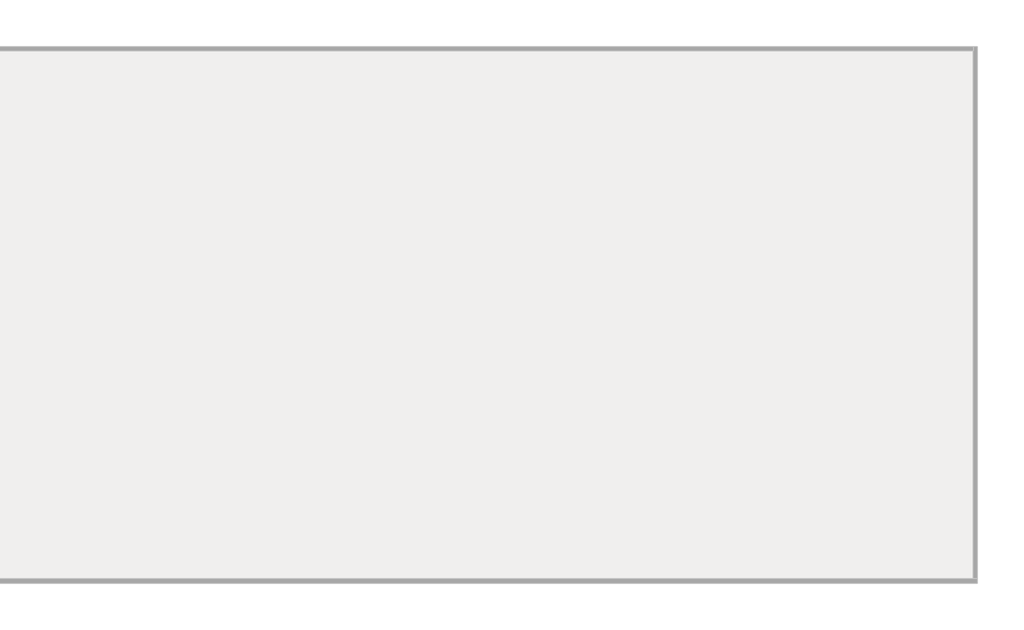
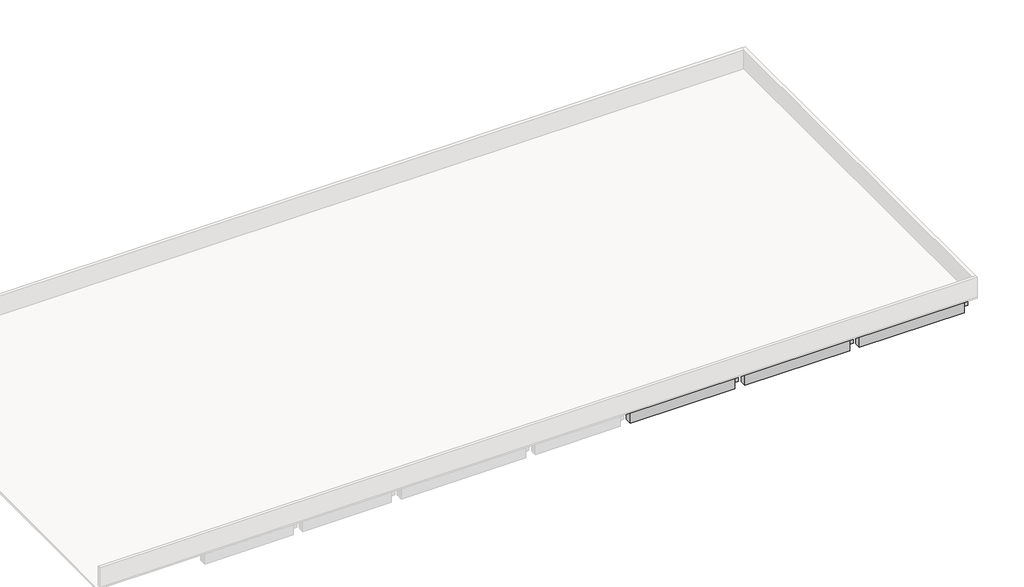
# One storey, part 2 of 2: 26 beams.
"""IFC4 building model written with IfcOpenShell, lengths in millimetres."""

from ifc_helpers import new_model, si_unit, origin, place, context, project, spatial, faceted_brep, element, save

model = new_model("IFC4")

# Units and contexts
model_context = context("Model", 3, world=origin())
ifc_project = project(units=[si_unit("LENGTHUNIT", "METRE", prefix="MILLI")], contexts=[model_context])

# Site, building, storey
site = spatial("IfcSite", under=ifc_project)
building = spatial("IfcBuilding", under=site)
storey = spatial("IfcBuildingStorey", under=building, Name="TOC", Elevation=7650.0)

# Beams
placement = place(None, origin())
element("IfcBeam", 1, ObjectType="RC Beam_Rectangular : H_SB_ACB_B400xH900", at=placement, inside=storey, context=model_context, shape_type="Brep", body=[
    faceted_brep([(39124.7, 12116.5208589, 6750.0), (39124.7, 12116.5208589, 7549.0), (38724.7, 12116.5208589, 7549.0), (33391.7, 12116.5208589, 7549.0), (33157.7, 12116.5208589, 7549.0), (32124.7, 12116.5208589, 7549.0), (32124.7, 12116.5208589, 6750.0), (33157.7, 12116.5208589, 6750.0), (33391.7, 12116.5208589, 6750.0), (38724.7, 12116.5208589, 6750.0), (39124.7, 12516.5208589, 6750.0), (32124.7, 12516.5208589, 6750.0), (33157.7, 12516.5208589, 6750.0), (33391.7, 12516.5208589, 6750.0), (38724.7, 12516.5208589, 6750.0), (39124.7, 12516.5208589, 7549.0), (32124.7, 12516.5208589, 7549.0), (33157.7, 12516.5208589, 7549.0), (33391.7, 12516.5208589, 7549.0), (38724.7, 12516.5208589, 7549.0)], [[[0, 1, 2, 3, 4, 5, 6, 7, 8, 9]], [[10, 0, 9, 8, 7, 6, 11, 12, 13, 14]], [[15, 10, 14, 13, 12, 11, 16, 17, 18, 19]], [[1, 15, 19, 18, 17, 16, 5, 4, 3, 2]], [[0, 10, 15, 1]], [[6, 5, 16, 11]]]),
])
element("IfcBeam", 2, ObjectType="RC Beam_Rectangular : H_SB_ACB_B400xH900", at=placement, inside=storey, context=model_context, shape_type="Brep", body=[
    faceted_brep([(46124.7, 12116.5208589, 6750.0), (46124.7, 12116.5208589, 7549.0), (45724.7, 12116.5208589, 7549.0), (43841.7, 12116.5208589, 7549.0), (43607.7, 12116.5208589, 7549.0), (39124.7, 12116.5208589, 7549.0), (39124.7, 12116.5208589, 6750.0), (43607.7, 12116.5208589, 6750.0), (43841.7, 12116.5208589, 6750.0), (45724.7, 12116.5208589, 6750.0), (46124.7, 12516.5208589, 6750.0), (39124.7, 12516.5208589, 6750.0), (43607.7, 12516.5208589, 6750.0), (43841.7, 12516.5208589, 6750.0), (45724.7, 12516.5208589, 6750.0), (46124.7, 12516.5208589, 7549.0), (39124.7, 12516.5208589, 7549.0), (43607.7, 12516.5208589, 7549.0), (43841.7, 12516.5208589, 7549.0), (45724.7, 12516.5208589, 7549.0)], [[[0, 1, 2, 3, 4, 5, 6, 7, 8, 9]], [[10, 0, 9, 8, 7, 6, 11, 12, 13, 14]], [[15, 10, 14, 13, 12, 11, 16, 17, 18, 19]], [[1, 15, 19, 18, 17, 16, 5, 4, 3, 2]], [[0, 10, 15, 1]], [[6, 5, 16, 11]]]),
])
element("IfcBeam", 3, ObjectType="RC Beam_Rectangular : H_SB_ACB_B400xH900", at=placement, inside=storey, context=model_context, shape_type="Brep", body=[
    faceted_brep([(53124.7, 12116.5208589, 6750.0), (53124.7, 12116.5208589, 7549.0), (52724.7, 12116.5208589, 7549.0), (46124.7, 12116.5208589, 7549.0), (46124.7, 12116.5208589, 6750.0), (52724.7, 12116.5208589, 6750.0), (53124.7, 12516.5208589, 6750.0), (46124.7, 12516.5208589, 6750.0), (52724.7, 12516.5208589, 6750.0), (53124.7, 12516.5208589, 7549.0), (46124.7, 12516.5208589, 7549.0), (52724.7, 12516.5208589, 7549.0)], [[[0, 1, 2, 3, 4, 5]], [[6, 0, 5, 4, 7, 8]], [[9, 6, 8, 7, 10, 11]], [[1, 9, 11, 10, 3, 2]], [[0, 6, 9, 1]], [[4, 3, 10, 7]]]),
])
element("IfcBeam", 4, ObjectType="RC Beam_Rectangular : H_SB_ACB_B400xH900", at=placement, inside=storey, context=model_context, shape_type="Brep", body=[
    faceted_brep([(18224.7, 23816.5208589, 7500.0), (18224.7, 23816.5208589, 6750.0), (25824.7, 23816.5208589, 6750.0), (25824.7, 23816.5208589, 7500.0), (25924.7, 23816.5208589, 7500.0), (25924.7, 23816.5208589, 7549.0), (18124.7, 23816.5208589, 7549.0), (18124.7, 23816.5208589, 7500.0), (18224.7, 23886.5208589, 6750.0), (18224.7, 24216.5208589, 6750.0), (25824.7, 24216.5208589, 6750.0), (25824.7, 23886.5208589, 6750.0), (18224.7, 24216.5208589, 7500.0), (18124.7, 24216.5208589, 7500.0), (18124.7, 24216.5208589, 7549.0), (25924.7, 24216.5208589, 7549.0), (25924.7, 24216.5208589, 7500.0), (25824.7, 24216.5208589, 7500.0)], [[[0, 1, 2, 3, 4, 5, 6, 7]], [[1, 8, 9, 10, 11, 2]], [[9, 12, 13, 14, 15, 16, 17, 10]], [[1, 0, 12, 9, 8]], [[0, 7, 13, 12]], [[3, 2, 11, 10, 17]], [[3, 17, 16, 4]], [[14, 6, 5, 15]], [[6, 14, 13, 7]], [[5, 4, 16, 15]]]),
])
element("IfcBeam", 5, ObjectType="RC Beam_Rectangular : H_SB_ACB_B400xH900", at=placement, inside=storey, context=model_context, shape_type="Brep", body=[
    faceted_brep([(26424.7, 23816.5208589, 7500.0), (26424.7, 23816.5208589, 6750.0), (31624.7, 23816.5208589, 6750.0), (31624.7, 23816.5208589, 7500.0), (31724.7, 23816.5208589, 7500.0), (31724.7, 23816.5208589, 7549.0), (26324.7, 23816.5208589, 7549.0), (26324.7, 23816.5208589, 7500.0), (26424.7, 23886.5208589, 6750.0), (26424.7, 24216.5208589, 6750.0), (31624.7, 24216.5208589, 6750.0), (31624.7, 23886.5208589, 6750.0), (26424.7, 24216.5208589, 7500.0), (26324.7, 24216.5208589, 7500.0), (26324.7, 24216.5208589, 7549.0), (31724.7, 24216.5208589, 7549.0), (31724.7, 24216.5208589, 7500.0), (31624.7, 24216.5208589, 7500.0)], [[[0, 1, 2, 3, 4, 5, 6, 7]], [[1, 8, 9, 10, 11, 2]], [[9, 12, 13, 14, 15, 16, 17, 10]], [[1, 0, 12, 9, 8]], [[0, 7, 13, 12]], [[3, 2, 11, 10, 17]], [[3, 17, 16, 4]], [[14, 6, 5, 15]], [[6, 14, 13, 7]], [[5, 4, 16, 15]]]),
])
element("IfcBeam", 6, ObjectType="RC Beam_Rectangular : H_SB_ACB_B400xH900", at=placement, inside=storey, context=model_context, shape_type="Brep", body=[
    faceted_brep([(32224.7, 23816.5208589, 7500.0), (32224.7, 23816.5208589, 6750.0), (33157.7, 23816.5208589, 6750.0), (33391.7, 23816.5208589, 6750.0), (38624.7, 23816.5208589, 6750.0), (38624.7, 23816.5208589, 7500.0), (38724.7, 23816.5208589, 7500.0), (38724.7, 23816.5208589, 7549.0), (33391.7, 23816.5208589, 7549.0), (33157.7, 23816.5208589, 7549.0), (32124.7, 23816.5208589, 7549.0), (32124.7, 23816.5208589, 7500.0), (32224.7, 23886.5208589, 6750.0), (32224.7, 24216.5208589, 6750.0), (38624.7, 24216.5208589, 6750.0), (38624.7, 23886.5208589, 6750.0), (32224.7, 24216.5208589, 7500.0), (32124.7, 24216.5208589, 7500.0), (32124.7, 24216.5208589, 7549.0), (38724.7, 24216.5208589, 7549.0), (38724.7, 24216.5208589, 7500.0), (38624.7, 24216.5208589, 7500.0)], [[[0, 1, 2, 3, 4, 5, 6, 7, 8, 9, 10, 11]], [[1, 12, 13, 14, 15, 4, 3, 2]], [[13, 16, 17, 18, 19, 20, 21, 14]], [[1, 0, 16, 13, 12]], [[0, 11, 17, 16]], [[5, 4, 15, 14, 21]], [[5, 21, 20, 6]], [[18, 10, 9, 8, 7, 19]], [[10, 18, 17, 11]], [[7, 6, 20, 19]]]),
])
element("IfcBeam", 7, ObjectType="RC Beam_Rectangular : H_SB_ACB_B400xH900", at=placement, inside=storey, context=model_context, shape_type="Brep", body=[
    faceted_brep([(39224.7, 23816.5208589, 7500.0), (39224.7, 23816.5208589, 6750.0), (43607.7, 23816.5208589, 6750.0), (43841.7, 23816.5208589, 6750.0), (45624.7, 23816.5208589, 6750.0), (45624.7, 23816.5208589, 7500.0), (45724.7, 23816.5208589, 7500.0), (45724.7, 23816.5208589, 7549.0), (43841.7, 23816.5208589, 7549.0), (43607.7, 23816.5208589, 7549.0), (39124.7, 23816.5208589, 7549.0), (39124.7, 23816.5208589, 7500.0), (39224.7, 23886.5208589, 6750.0), (39224.7, 24216.5208589, 6750.0), (45624.7, 24216.5208589, 6750.0), (45624.7, 23886.5208589, 6750.0), (39224.7, 24216.5208589, 7500.0), (39124.7, 24216.5208589, 7500.0), (39124.7, 24216.5208589, 7549.0), (45724.7, 24216.5208589, 7549.0), (45724.7, 24216.5208589, 7500.0), (45624.7, 24216.5208589, 7500.0)], [[[0, 1, 2, 3, 4, 5, 6, 7, 8, 9, 10, 11]], [[1, 12, 13, 14, 15, 4, 3, 2]], [[13, 16, 17, 18, 19, 20, 21, 14]], [[1, 0, 16, 13, 12]], [[0, 11, 17, 16]], [[5, 4, 15, 14, 21]], [[5, 21, 20, 6]], [[18, 10, 9, 8, 7, 19]], [[10, 18, 17, 11]], [[7, 6, 20, 19]]]),
])
element("IfcBeam", 8, ObjectType="RC Beam_Rectangular : H_SB_ACB_B400xH900", at=placement, inside=storey, context=model_context, shape_type="Brep", body=[
    faceted_brep([(46224.7, 23816.5208589, 7500.0), (46224.7, 23816.5208589, 6750.0), (48807.7, 23816.5208589, 6750.0), (49041.7, 23816.5208589, 6750.0), (52624.7, 23816.5208589, 6750.0), (52624.7, 23816.5208589, 7500.0), (52724.7, 23816.5208589, 7500.0), (52724.7, 23816.5208589, 7549.0), (49041.7, 23816.5208589, 7549.0), (48807.7, 23816.5208589, 7549.0), (46124.7, 23816.5208589, 7549.0), (46124.7, 23816.5208589, 7500.0), (46224.7, 23886.5208589, 6750.0), (46224.7, 24216.5208589, 6750.0), (52624.7, 24216.5208589, 6750.0), (52624.7, 23886.5208589, 6750.0), (46224.7, 24216.5208589, 7500.0), (46124.7, 24216.5208589, 7500.0), (46124.7, 24216.5208589, 7549.0), (52724.7, 24216.5208589, 7549.0), (52724.7, 24216.5208589, 7500.0), (52624.7, 24216.5208589, 7500.0)], [[[0, 1, 2, 3, 4, 5, 6, 7, 8, 9, 10, 11]], [[1, 12, 13, 14, 15, 4, 3, 2]], [[13, 16, 17, 18, 19, 20, 21, 14]], [[1, 0, 16, 13, 12]], [[0, 11, 17, 16]], [[5, 4, 15, 14, 21]], [[5, 21, 20, 6]], [[18, 10, 9, 8, 7, 19]], [[10, 18, 17, 11]], [[7, 6, 20, 19]]]),
])
element("IfcBeam", 9, ObjectType="RC Beam_Rectangular : H_SB_ACB_B400xH900", at=placement, inside=storey, context=model_context, shape_type="Brep", body=[
    faceted_brep([(32224.7, 8216.5208589, 7500.0), (32224.7, 8216.5208589, 6750.0), (36207.7, 8216.5208589, 6750.0), (36441.7, 8216.5208589, 6750.0), (38624.7, 8216.5208589, 6750.0), (38624.7, 8216.5208589, 7500.0), (38724.7, 8216.5208589, 7500.0), (39124.7, 8216.5208589, 7500.0), (39124.7, 8216.5208589, 7549.0), (38724.7, 8216.5208589, 7549.0), (36441.7, 8216.5208589, 7549.0), (36207.7, 8216.5208589, 7549.0), (32124.7, 8216.5208589, 7549.0), (32124.7, 8216.5208589, 7500.0), (32224.7, 8299.5208589, 6750.0), (32224.7, 8533.5208589, 6750.0), (32224.7, 8616.5208589, 6750.0), (33157.7, 8616.5208589, 6750.0), (33391.7, 8616.5208589, 6750.0), (36207.7, 8616.5208589, 6750.0), (36441.7, 8616.5208589, 6750.0), (38624.7, 8616.5208589, 6750.0), (32224.7, 8616.5208589, 7500.0), (32124.7, 8616.5208589, 7500.0), (32124.7, 8616.5208589, 7549.0), (33157.7, 8616.5208589, 7549.0), (33391.7, 8616.5208589, 7549.0), (36207.7, 8616.5208589, 7549.0), (36441.7, 8616.5208589, 7549.0), (38724.7, 8616.5208589, 7549.0), (39124.7, 8616.5208589, 7549.0), (39124.7, 8616.5208589, 7500.0), (38724.7, 8616.5208589, 7500.0), (38624.7, 8616.5208589, 7500.0)], [[[0, 1, 2, 3, 4, 5, 6, 7, 8, 9, 10, 11, 12, 13]], [[1, 14, 15, 16, 17, 18, 19, 20, 21, 4, 3, 2]], [[16, 22, 23, 24, 25, 26, 27, 28, 29, 30, 31, 32, 33, 21, 20, 19, 18, 17]], [[1, 0, 22, 16, 15, 14]], [[0, 13, 23, 22]], [[33, 5, 4, 21]], [[5, 33, 32, 31, 7, 6]], [[12, 11, 10, 9, 8, 30, 29, 28, 27, 26, 25, 24]], [[30, 8, 7, 31]], [[12, 24, 23, 13]]]),
])
element("IfcBeam", 10, ObjectType="RC Beam_Rectangular : H_SB_ACB_B400xH900", at=placement, inside=storey, context=model_context, shape_type="Brep", body=[
    faceted_brep([(39224.7, 8216.5208589, 7500.0), (39224.7, 8216.5208589, 6750.0), (41890.7, 8216.5208589, 6750.0), (42124.7, 8216.5208589, 6750.0), (43107.7, 8216.5208589, 6750.0), (43341.7, 8216.5208589, 6750.0), (45175.8778017, 8216.5208589, 6750.0), (45409.8778017, 8216.5208589, 6750.0), (45624.7, 8216.5208589, 6750.0), (45624.7, 8216.5208589, 7500.0), (45724.7, 8216.5208589, 7500.0), (46124.7, 8216.5208589, 7500.0), (46124.7, 8216.5208589, 7549.0), (45724.7, 8216.5208589, 7549.0), (45409.8778017, 8216.5208589, 7549.0), (45175.8778017, 8216.5208589, 7549.0), (43341.7, 8216.5208589, 7549.0), (43107.7, 8216.5208589, 7549.0), (42124.7, 8216.5208589, 7549.0), (41890.7, 8216.5208589, 7549.0), (39124.7, 8216.5208589, 7549.0), (39124.7, 8216.5208589, 7500.0), (39224.7, 8299.5208589, 6750.0), (39224.7, 8533.5208589, 6750.0), (39224.7, 8616.5208589, 6750.0), (45624.7, 8616.5208589, 6750.0), (45624.7, 8533.5208589, 6750.0), (45624.7, 8299.5208589, 6750.0), (39224.7, 8616.5208589, 7500.0), (39124.7, 8616.5208589, 7500.0), (39124.7, 8616.5208589, 7549.0), (45724.7, 8616.5208589, 7549.0), (46124.7, 8616.5208589, 7549.0), (46124.7, 8616.5208589, 7500.0), (45724.7, 8616.5208589, 7500.0), (45624.7, 8616.5208589, 7500.0)], [[[0, 1, 2, 3, 4, 5, 6, 7, 8, 9, 10, 11, 12, 13, 14, 15, 16, 17, 18, 19, 20, 21]], [[1, 22, 23, 24, 25, 26, 27, 8, 7, 6, 5, 4, 3, 2]], [[24, 28, 29, 30, 31, 32, 33, 34, 35, 25]], [[1, 0, 28, 24, 23, 22]], [[0, 21, 29, 28]], [[35, 9, 8, 27, 26, 25]], [[9, 35, 34, 33, 11, 10]], [[20, 19, 18, 17, 16, 15, 14, 13, 12, 32, 31, 30]], [[32, 12, 11, 33]], [[20, 30, 29, 21]]]),
])
element("IfcBeam", 11, ObjectType="RC Beam_Rectangular : H_SB_ACB_B400xH900", at=placement, inside=storey, context=model_context, shape_type="Brep", body=[
    faceted_brep([(46224.7, 8216.5208589, 7500.0), (46224.7, 8216.5208589, 6750.0), (52624.7, 8216.5208589, 6750.0), (52624.7, 8216.5208589, 7500.0), (52724.7, 8216.5208589, 7500.0), (53124.7, 8216.5208589, 7500.0), (53124.7, 8216.5208589, 7549.0), (52724.7, 8216.5208589, 7549.0), (46124.7, 8216.5208589, 7549.0), (46124.7, 8216.5208589, 7500.0), (46224.7, 8299.5208589, 6750.0), (46224.7, 8533.5208589, 6750.0), (46224.7, 8616.5208589, 6750.0), (50660.7, 8616.5208589, 6750.0), (50894.7, 8616.5208589, 6750.0), (52624.7, 8616.5208589, 6750.0), (52624.7, 8533.5208589, 6750.0), (52624.7, 8299.5208589, 6750.0), (46224.7, 8616.5208589, 7500.0), (46124.7, 8616.5208589, 7500.0), (46124.7, 8616.5208589, 7549.0), (50660.7, 8616.5208589, 7549.0), (50894.7, 8616.5208589, 7549.0), (52724.7, 8616.5208589, 7549.0), (53124.7, 8616.5208589, 7549.0), (53124.7, 8616.5208589, 7500.0), (52724.7, 8616.5208589, 7500.0), (52624.7, 8616.5208589, 7500.0)], [[[0, 1, 2, 3, 4, 5, 6, 7, 8, 9]], [[1, 10, 11, 12, 13, 14, 15, 16, 17, 2]], [[12, 18, 19, 20, 21, 22, 23, 24, 25, 26, 27, 15, 14, 13]], [[1, 0, 18, 12, 11, 10]], [[0, 9, 19, 18]], [[27, 3, 2, 17, 16, 15]], [[3, 27, 26, 25, 5, 4]], [[8, 7, 6, 24, 23, 22, 21, 20]], [[24, 6, 5, 25]], [[8, 20, 19, 9]]]),
])
element("IfcBeam", 12, ObjectType="RC Beam_Rectangular : H_SB_ACB_B400xH900", at=placement, inside=storey, context=model_context, shape_type="Brep", body=[
    faceted_brep([(32224.7, 416.5208589, 7500.0), (32224.7, 416.5208589, 6750.0), (38624.7, 416.5208589, 6750.0), (38624.7, 416.5208589, 7500.0), (39124.7, 416.5208589, 7500.0), (39124.7, 416.5208589, 7549.0), (32124.7, 416.5208589, 7549.0), (32124.7, 416.5208589, 7500.0), (32224.7, 746.5208589, 6750.0), (32224.7, 816.5208589, 6750.0), (36207.7, 816.5208589, 6750.0), (36441.7, 816.5208589, 6750.0), (38624.7, 816.5208589, 6750.0), (38624.7, 746.5208589, 6750.0), (32224.7, 816.5208589, 7500.0), (32124.7, 816.5208589, 7500.0), (32124.7, 816.5208589, 7549.0), (36207.7, 816.5208589, 7549.0), (36441.7, 816.5208589, 7549.0), (38724.7, 816.5208589, 7549.0), (39124.7, 816.5208589, 7549.0), (39124.7, 816.5208589, 7500.0), (38724.7, 816.5208589, 7500.0), (38624.7, 816.5208589, 7500.0)], [[[0, 1, 2, 3, 4, 5, 6, 7]], [[1, 8, 9, 10, 11, 12, 13, 2]], [[9, 14, 15, 16, 17, 18, 19, 20, 21, 22, 23, 12, 11, 10]], [[9, 8, 1, 0, 14]], [[15, 14, 0, 7]], [[23, 3, 2, 13, 12]], [[3, 23, 22, 21, 4]], [[6, 5, 20, 19, 18, 17, 16]], [[20, 5, 4, 21]], [[6, 16, 15, 7]]]),
])
element("IfcBeam", 13, ObjectType="RC Beam_Rectangular : H_SB_ACB_B400xH900", at=placement, inside=storey, context=model_context, shape_type="Brep", body=[
    faceted_brep([(39224.7, 416.5208589, 7500.0), (39224.7, 416.5208589, 6750.0), (45624.7, 416.5208589, 6750.0), (45624.7, 416.5208589, 7500.0), (46124.7, 416.5208589, 7500.0), (46124.7, 416.5208589, 7549.0), (39124.7, 416.5208589, 7549.0), (39124.7, 416.5208589, 7500.0), (39224.7, 746.5208589, 6750.0), (39224.7, 816.5208589, 6750.0), (43107.7, 816.5208589, 6750.0), (43341.7, 816.5208589, 6750.0), (45624.7, 816.5208589, 6750.0), (45624.7, 746.5208589, 6750.0), (39224.7, 816.5208589, 7500.0), (39124.7, 816.5208589, 7500.0), (39124.7, 816.5208589, 7549.0), (43107.7, 816.5208589, 7549.0), (43341.7, 816.5208589, 7549.0), (45724.7, 816.5208589, 7549.0), (46124.7, 816.5208589, 7549.0), (46124.7, 816.5208589, 7500.0), (45724.7, 816.5208589, 7500.0), (45624.7, 816.5208589, 7500.0)], [[[0, 1, 2, 3, 4, 5, 6, 7]], [[1, 8, 9, 10, 11, 12, 13, 2]], [[9, 14, 15, 16, 17, 18, 19, 20, 21, 22, 23, 12, 11, 10]], [[9, 8, 1, 0, 14]], [[15, 14, 0, 7]], [[23, 3, 2, 13, 12]], [[3, 23, 22, 21, 4]], [[6, 5, 20, 19, 18, 17, 16]], [[20, 5, 4, 21]], [[6, 16, 15, 7]]]),
])
element("IfcBeam", 14, ObjectType="RC Beam_Rectangular : H_SB_ACB_B400xH900", at=placement, inside=storey, context=model_context, shape_type="Brep", body=[
    faceted_brep([(46224.7, 416.5208589, 7500.0), (46224.7, 416.5208589, 6750.0), (52624.7, 416.5208589, 6750.0), (52624.7, 416.5208589, 7500.0), (53124.7, 416.5208589, 7500.0), (53124.7, 416.5208589, 7549.0), (46124.7, 416.5208589, 7549.0), (46124.7, 416.5208589, 7500.0), (46224.7, 746.5208589, 6750.0), (46224.7, 816.5208589, 6750.0), (46507.7, 816.5208589, 6750.0), (46741.7, 816.5208589, 6750.0), (52624.7, 816.5208589, 6750.0), (52624.7, 746.5208589, 6750.0), (46224.7, 816.5208589, 7500.0), (46124.7, 816.5208589, 7500.0), (46124.7, 816.5208589, 7549.0), (46507.7, 816.5208589, 7549.0), (46741.7, 816.5208589, 7549.0), (52724.7, 816.5208589, 7549.0), (53124.7, 816.5208589, 7549.0), (53124.7, 816.5208589, 7500.0), (52724.7, 816.5208589, 7500.0), (52624.7, 816.5208589, 7500.0), (53124.7, 746.5208589, 7500.0), (53124.7, 746.5208589, 7549.0)], [[[0, 1, 2, 3, 4, 5, 6, 7]], [[1, 8, 9, 10, 11, 12, 13, 2]], [[9, 14, 15, 16, 17, 18, 19, 20, 21, 22, 23, 12, 11, 10]], [[9, 8, 1, 0, 14]], [[15, 14, 0, 7]], [[23, 3, 2, 13, 12]], [[3, 23, 22, 21, 24, 4]], [[6, 5, 25, 20, 19, 18, 17, 16]], [[20, 25, 5, 4, 24, 21]], [[6, 16, 15, 7]]]),
])
element("IfcBeam", 15, ObjectType="RC Beam_Rectangular : H_SB_ACB_B400xH900", at=placement, inside=storey, context=model_context, shape_type="Brep", body=[
    faceted_brep([(18124.7, 24429.2208589, 6750.0), (17724.7, 24429.2208589, 6750.0), (17724.7, 24429.2208589, 7549.0), (18124.7, 24429.2208589, 7549.0), (18124.7, 12616.5208589, 7500.0), (18124.7, 12616.5208589, 6750.0), (18124.7, 23716.5208589, 6750.0), (18124.7, 23716.5208589, 7500.0), (18124.7, 23816.5208589, 7500.0), (18124.7, 24216.5208589, 7500.0), (18124.7, 24316.5208589, 7500.0), (18124.7, 24316.5208589, 6750.0), (18124.7, 24316.5208589, 7549.0), (18124.7, 24216.5208589, 7549.0), (18124.7, 23816.5208589, 7549.0), (18124.7, 12516.5208589, 7549.0), (18124.7, 12516.5208589, 7500.0), (17724.7, 24316.5208589, 6750.0), (17724.7, 24316.5208589, 7500.0), (17724.7, 24216.5208589, 7500.0), (17724.7, 23816.5208589, 7500.0), (17724.7, 23716.5208589, 7500.0), (17724.7, 23716.5208589, 6750.0), (17724.7, 12616.5208589, 6750.0), (17724.7, 12616.5208589, 7500.0), (17724.7, 12516.5208589, 7500.0), (17724.7, 12516.5208589, 7549.0), (17724.7, 23816.5208589, 7549.0), (17724.7, 24216.5208589, 7549.0), (17724.7, 24316.5208589, 7549.0), (17807.7, 12616.5208589, 6750.0), (18041.7, 12616.5208589, 6750.0), (18041.7, 23716.5208589, 6750.0), (17807.7, 23716.5208589, 6750.0)], [[[0, 1, 2, 3]], [[4, 5, 6, 7, 8, 9, 10, 11, 0, 3, 12, 13, 14, 15, 16]], [[1, 0, 11, 17]], [[2, 1, 17, 18, 19, 20, 21, 22, 23, 24, 25, 26, 27, 28, 29]], [[25, 16, 15, 26]], [[5, 4, 24, 23, 30, 31]], [[4, 16, 25, 24]], [[21, 7, 6, 32, 33, 22]], [[7, 21, 20, 19, 18, 10, 9, 8]], [[3, 2, 29, 28, 27, 26, 15, 14, 13, 12]], [[10, 18, 17, 11]], [[5, 31, 30, 23, 22, 33, 32, 6]]]),
])
element("IfcBeam", 16, ObjectType="RC Beam_Rectangular : H_SB_ACB_B400xH900", at=placement, inside=storey, context=model_context, shape_type="Brep", body=[
    faceted_brep([(26324.7, 24429.2208589, 6750.0), (25924.7, 24429.2208589, 6750.0), (25924.7, 24429.2208589, 7549.0), (26324.7, 24429.2208589, 7549.0), (26324.7, 24316.5208589, 7549.0), (26324.7, 24216.5208589, 7549.0), (26324.7, 23816.5208589, 7549.0), (26324.7, 12516.5208589, 7549.0), (26324.7, 12516.5208589, 6750.0), (26324.7, 23716.5208589, 6750.0), (26324.7, 23716.5208589, 7500.0), (26324.7, 23816.5208589, 7500.0), (26324.7, 24216.5208589, 7500.0), (26324.7, 24316.5208589, 7500.0), (26324.7, 24316.5208589, 6750.0), (25924.7, 24316.5208589, 6750.0), (25924.7, 12516.5208589, 6750.0), (25924.7, 12516.5208589, 7549.0), (25924.7, 23816.5208589, 7549.0), (25924.7, 24216.5208589, 7549.0), (25924.7, 24316.5208589, 7549.0), (25924.7, 24316.5208589, 7500.0), (25924.7, 24216.5208589, 7500.0), (25924.7, 23816.5208589, 7500.0), (25924.7, 23716.5208589, 7500.0), (25924.7, 23716.5208589, 6750.0)], [[[0, 1, 2, 3]], [[0, 3, 4, 5, 6, 7, 8, 9, 10, 11, 12, 13, 14]], [[1, 0, 14, 15]], [[16, 17, 18, 19, 20, 2, 1, 15, 21, 22, 23, 24, 25]], [[16, 8, 7, 17]], [[24, 10, 9, 25]], [[10, 24, 23, 22, 21, 13, 12, 11]], [[3, 2, 20, 19, 18, 17, 7, 6, 5, 4]], [[13, 21, 15, 14]], [[8, 16, 25, 9]]]),
])
element("IfcBeam", 17, ObjectType="RC Beam_Rectangular : H_SB_ACB_B400xH900", at=placement, inside=storey, context=model_context, shape_type="Brep", body=[
    faceted_brep([(32124.7, 24429.2208589, 6750.0), (31724.7, 24429.2208589, 6750.0), (31724.7, 24429.2208589, 7549.0), (32124.7, 24429.2208589, 7549.0), (32124.7, 24316.5208589, 7549.0), (32124.7, 24216.5208589, 7549.0), (32124.7, 23816.5208589, 7549.0), (32124.7, 12516.5208589, 7549.0), (32124.7, 12516.5208589, 6750.0), (32124.7, 23716.5208589, 6750.0), (32124.7, 23716.5208589, 7500.0), (32124.7, 23816.5208589, 7500.0), (32124.7, 24216.5208589, 7500.0), (32124.7, 24316.5208589, 7500.0), (32124.7, 24316.5208589, 6750.0), (31724.7, 24316.5208589, 6750.0), (31724.7, 12516.5208589, 6750.0), (31724.7, 12516.5208589, 7549.0), (31724.7, 23816.5208589, 7549.0), (31724.7, 24216.5208589, 7549.0), (31724.7, 24316.5208589, 7549.0), (31724.7, 24316.5208589, 7500.0), (31724.7, 24216.5208589, 7500.0), (31724.7, 23816.5208589, 7500.0), (31724.7, 23716.5208589, 7500.0), (31724.7, 23716.5208589, 6750.0)], [[[0, 1, 2, 3]], [[0, 3, 4, 5, 6, 7, 8, 9, 10, 11, 12, 13, 14]], [[1, 0, 14, 15]], [[16, 17, 18, 19, 20, 2, 1, 15, 21, 22, 23, 24, 25]], [[16, 8, 7, 17]], [[24, 10, 9, 25]], [[10, 24, 23, 22, 21, 13, 12, 11]], [[3, 2, 20, 19, 18, 17, 7, 6, 5, 4]], [[13, 21, 15, 14]], [[8, 16, 25, 9]]]),
])
element("IfcBeam", 18, ObjectType="RC Beam_Rectangular : H_SB_ACB_B400xH900", at=placement, inside=storey, context=model_context, shape_type="Brep", body=[
    faceted_brep([(39124.7, 8116.5208589, 6750.0), (39124.7, 8116.5208589, 7500.0), (39124.7, 8216.5208589, 7500.0), (39124.7, 8216.5208589, 7549.0), (39124.7, 7080.5208589, 7549.0), (39124.7, 6846.5208589, 7549.0), (39124.7, 5130.5208589, 7549.0), (39124.7, 4896.5208589, 7549.0), (39124.7, 816.5208589, 7549.0), (39124.7, 816.5208589, 7500.0), (39124.7, 916.5208589, 7500.0), (39124.7, 916.5208589, 6750.0), (39124.7, 4896.5208589, 6750.0), (39124.7, 5130.5208589, 6750.0), (39124.7, 6846.5208589, 6750.0), (39124.7, 7080.5208589, 6750.0), (38724.7, 8116.5208589, 6750.0), (38807.7, 8116.5208589, 6750.0), (39041.7, 8116.5208589, 6750.0), (39041.7, 916.5208589, 6750.0), (38807.7, 916.5208589, 6750.0), (38724.7, 916.5208589, 6750.0), (38724.7, 3146.5208589, 6750.0), (38724.7, 3380.5208589, 6750.0), (38724.7, 8116.5208589, 7500.0), (38724.7, 916.5208589, 7500.0), (38724.7, 816.5208589, 7500.0), (38724.7, 816.5208589, 7549.0), (38724.7, 3146.5208589, 7549.0), (38724.7, 3380.5208589, 7549.0), (38724.7, 8216.5208589, 7549.0), (38724.7, 8216.5208589, 7500.0)], [[[0, 1, 2, 3, 4, 5, 6, 7, 8, 9, 10, 11, 12, 13, 14, 15]], [[16, 17, 18, 0, 15, 14, 13, 12, 11, 19, 20, 21, 22, 23]], [[24, 16, 23, 22, 21, 25, 26, 27, 28, 29, 30, 31]], [[2, 31, 30, 3]], [[8, 27, 26, 9]], [[1, 0, 18, 17, 16, 24]], [[2, 1, 24, 31]], [[10, 25, 21, 20, 19, 11]], [[25, 10, 9, 26]], [[3, 30, 29, 28, 27, 8, 7, 6, 5, 4]]]),
])
element("IfcBeam", 19, ObjectType="RC Beam_Rectangular : H_SB_ACB_B400xH900", at=placement, inside=storey, context=model_context, shape_type="Brep", body=[
    faceted_brep([(39124.7, 12116.5208589, 6750.0), (39124.7, 12116.5208589, 7549.0), (39124.7, 11083.5208589, 7549.0), (39124.7, 10849.5208589, 7549.0), (39124.7, 8616.5208589, 7549.0), (39124.7, 8616.5208589, 7500.0), (39124.7, 8716.5208589, 7500.0), (39124.7, 8716.5208589, 6750.0), (39124.7, 10849.5208589, 6750.0), (39124.7, 11083.5208589, 6750.0), (38724.7, 12116.5208589, 6750.0), (38724.7, 8716.5208589, 6750.0), (38724.7, 10849.5208589, 6750.0), (38724.7, 11083.5208589, 6750.0), (38724.7, 12116.5208589, 7549.0), (38724.7, 8716.5208589, 7500.0), (38724.7, 8616.5208589, 7500.0), (38724.7, 8616.5208589, 7549.0), (38724.7, 10849.5208589, 7549.0), (38724.7, 11083.5208589, 7549.0)], [[[0, 1, 2, 3, 4, 5, 6, 7, 8, 9]], [[10, 0, 9, 8, 7, 11, 12, 13]], [[14, 10, 13, 12, 11, 15, 16, 17, 18, 19]], [[0, 10, 14, 1]], [[4, 17, 16, 5]], [[6, 15, 11, 7]], [[15, 6, 5, 16]], [[1, 14, 19, 18, 17, 4, 3, 2]]]),
])
element("IfcBeam", 20, ObjectType="RC Beam_Rectangular : H_SB_ACB_B400xH900", at=placement, inside=storey, context=model_context, shape_type="Brep", body=[
    faceted_brep([(39124.7, 24429.2208589, 6750.0), (38724.7, 24429.2208589, 6750.0), (38724.7, 24429.2208589, 7549.0), (39124.7, 24429.2208589, 7549.0), (39124.7, 24316.5208589, 7549.0), (39124.7, 24216.5208589, 7549.0), (39124.7, 23816.5208589, 7549.0), (39124.7, 12516.5208589, 7549.0), (39124.7, 12516.5208589, 6750.0), (39124.7, 23716.5208589, 6750.0), (39124.7, 23716.5208589, 7500.0), (39124.7, 23816.5208589, 7500.0), (39124.7, 24216.5208589, 7500.0), (39124.7, 24316.5208589, 7500.0), (39124.7, 24316.5208589, 6750.0), (38724.7, 24316.5208589, 6750.0), (38724.7, 12516.5208589, 6750.0), (38724.7, 12516.5208589, 7549.0), (38724.7, 23816.5208589, 7549.0), (38724.7, 24216.5208589, 7549.0), (38724.7, 24316.5208589, 7549.0), (38724.7, 24316.5208589, 7500.0), (38724.7, 24216.5208589, 7500.0), (38724.7, 23816.5208589, 7500.0), (38724.7, 23716.5208589, 7500.0), (38724.7, 23716.5208589, 6750.0)], [[[0, 1, 2, 3]], [[0, 3, 4, 5, 6, 7, 8, 9, 10, 11, 12, 13, 14]], [[1, 0, 14, 15]], [[16, 17, 18, 19, 20, 2, 1, 15, 21, 22, 23, 24, 25]], [[16, 8, 7, 17]], [[24, 10, 9, 25]], [[10, 24, 23, 22, 21, 13, 12, 11]], [[3, 2, 20, 19, 18, 17, 7, 6, 5, 4]], [[13, 21, 15, 14]], [[8, 16, 25, 9]]]),
])
element("IfcBeam", 21, ObjectType="RC Beam_Rectangular : H_SB_ACB_B400xH900", at=placement, inside=storey, context=model_context, shape_type="Brep", body=[
    faceted_brep([(46124.7, 8116.5208589, 6750.0), (46124.7, 8116.5208589, 7500.0), (46124.7, 8216.5208589, 7500.0), (46124.7, 8216.5208589, 7549.0), (46124.7, 6933.5208589, 7549.0), (46124.7, 6699.5208589, 7549.0), (46124.7, 5130.5208589, 7549.0), (46124.7, 4896.5208589, 7549.0), (46124.7, 816.5208589, 7549.0), (46124.7, 816.5208589, 7500.0), (46124.7, 916.5208589, 7500.0), (46124.7, 916.5208589, 6750.0), (46124.7, 4896.5208589, 6750.0), (46124.7, 5130.5208589, 6750.0), (46124.7, 6699.5208589, 6750.0), (46124.7, 6933.5208589, 6750.0), (45724.7, 8116.5208589, 6750.0), (45724.7, 916.5208589, 6750.0), (45724.7, 4896.5208589, 6750.0), (45724.7, 5130.5208589, 6750.0), (45724.7, 6699.5208589, 6750.0), (45724.7, 6933.5208589, 6750.0), (45724.7, 8116.5208589, 7500.0), (45724.7, 916.5208589, 7500.0), (45724.7, 816.5208589, 7500.0), (45724.7, 816.5208589, 7549.0), (45724.7, 4896.5208589, 7549.0), (45724.7, 5130.5208589, 7549.0), (45724.7, 6699.5208589, 7549.0), (45724.7, 6933.5208589, 7549.0), (45724.7, 8216.5208589, 7549.0), (45724.7, 8216.5208589, 7500.0)], [[[0, 1, 2, 3, 4, 5, 6, 7, 8, 9, 10, 11, 12, 13, 14, 15]], [[16, 0, 15, 14, 13, 12, 11, 17, 18, 19, 20, 21]], [[22, 16, 21, 20, 19, 18, 17, 23, 24, 25, 26, 27, 28, 29, 30, 31]], [[2, 31, 30, 3]], [[8, 25, 24, 9]], [[1, 0, 16, 22]], [[2, 1, 22, 31]], [[10, 23, 17, 11]], [[23, 10, 9, 24]], [[3, 30, 29, 28, 27, 26, 25, 8, 7, 6, 5, 4]]]),
])
element("IfcBeam", 22, ObjectType="RC Beam_Rectangular : H_SB_ACB_B400xH900", at=placement, inside=storey, context=model_context, shape_type="Brep", body=[
    faceted_brep([(46124.7, 12116.5208589, 6750.0), (46124.7, 12116.5208589, 7549.0), (46124.7, 10133.5208589, 7549.0), (46124.7, 9899.5208589, 7549.0), (46124.7, 8616.5208589, 7549.0), (46124.7, 8616.5208589, 7500.0), (46124.7, 8716.5208589, 7500.0), (46124.7, 8716.5208589, 6750.0), (46124.7, 9899.5208589, 6750.0), (46124.7, 10133.5208589, 6750.0), (45724.7, 12116.5208589, 6750.0), (45724.7, 8716.5208589, 6750.0), (45724.7, 10849.5208589, 6750.0), (45724.7, 11083.5208589, 6750.0), (45724.7, 12116.5208589, 7549.0), (45724.7, 8716.5208589, 7500.0), (45724.7, 8616.5208589, 7500.0), (45724.7, 8616.5208589, 7549.0), (45724.7, 10849.5208589, 7549.0), (45724.7, 11083.5208589, 7549.0)], [[[0, 1, 2, 3, 4, 5, 6, 7, 8, 9]], [[10, 0, 9, 8, 7, 11, 12, 13]], [[14, 10, 13, 12, 11, 15, 16, 17, 18, 19]], [[0, 10, 14, 1]], [[4, 17, 16, 5]], [[6, 15, 11, 7]], [[15, 6, 5, 16]], [[1, 14, 19, 18, 17, 4, 3, 2]]]),
])
element("IfcBeam", 23, ObjectType="RC Beam_Rectangular : H_SB_ACB_B400xH900", at=placement, inside=storey, context=model_context, shape_type="Brep", body=[
    faceted_brep([(46124.7, 24429.2208589, 6750.0), (45724.7, 24429.2208589, 6750.0), (45724.7, 24429.2208589, 7549.0), (46124.7, 24429.2208589, 7549.0), (46124.7, 24316.5208589, 7549.0), (46124.7, 24216.5208589, 7549.0), (46124.7, 23816.5208589, 7549.0), (46124.7, 20183.5208589, 7549.0), (46124.7, 19949.5208589, 7549.0), (46124.7, 18783.5208589, 7549.0), (46124.7, 18549.5208589, 7549.0), (46124.7, 17180.5208589, 7549.0), (46124.7, 16946.5208589, 7549.0), (46124.7, 15754.2234045, 7549.0), (46124.7, 15520.2234045, 7549.0), (46124.7, 14283.5208589, 7549.0), (46124.7, 14049.5208589, 7549.0), (46124.7, 12516.5208589, 7549.0), (46124.7, 12516.5208589, 6750.0), (46124.7, 14049.5208589, 6750.0), (46124.7, 14283.5208589, 6750.0), (46124.7, 15520.2234045, 6750.0), (46124.7, 15754.2234045, 6750.0), (46124.7, 16946.5208589, 6750.0), (46124.7, 17180.5208589, 6750.0), (46124.7, 18549.5208589, 6750.0), (46124.7, 18783.5208589, 6750.0), (46124.7, 19949.5208589, 6750.0), (46124.7, 20183.5208589, 6750.0), (46124.7, 23716.5208589, 6750.0), (46124.7, 23716.5208589, 7500.0), (46124.7, 23816.5208589, 7500.0), (46124.7, 24216.5208589, 7500.0), (46124.7, 24316.5208589, 7500.0), (46124.7, 24316.5208589, 6750.0), (45724.7, 24316.5208589, 6750.0), (45724.7, 12516.5208589, 6750.0), (45724.7, 12516.5208589, 7549.0), (45724.7, 21352.5208589, 7549.0), (45724.7, 21586.5208589, 7549.0), (45724.7, 23816.5208589, 7549.0), (45724.7, 24216.5208589, 7549.0), (45724.7, 24316.5208589, 7549.0), (45724.7, 24316.5208589, 7500.0), (45724.7, 24216.5208589, 7500.0), (45724.7, 23816.5208589, 7500.0), (45724.7, 23716.5208589, 7500.0), (45724.7, 23716.5208589, 6750.0), (45724.7, 21586.5208589, 6750.0), (45724.7, 21352.5208589, 6750.0), (46041.7, 23716.5208589, 6750.0), (45807.7, 23716.5208589, 6750.0)], [[[0, 1, 2, 3]], [[0, 3, 4, 5, 6, 7, 8, 9, 10, 11, 12, 13, 14, 15, 16, 17, 18, 19, 20, 21, 22, 23, 24, 25, 26, 27, 28, 29, 30, 31, 32, 33, 34]], [[1, 0, 34, 35]], [[36, 37, 38, 39, 40, 41, 42, 2, 1, 35, 43, 44, 45, 46, 47, 48, 49]], [[36, 18, 17, 37]], [[46, 30, 29, 50, 51, 47]], [[30, 46, 45, 44, 43, 33, 32, 31]], [[3, 2, 42, 41, 40, 39, 38, 37, 17, 16, 15, 14, 13, 12, 11, 10, 9, 8, 7, 6, 5, 4]], [[33, 43, 35, 34]], [[18, 36, 49, 48, 47, 51, 50, 29, 28, 27, 26, 25, 24, 23, 22, 21, 20, 19]]]),
])
element("IfcBeam", 24, ObjectType="RC Beam_Rectangular : H_SB_ACB_B400xH900", at=placement, inside=storey, context=model_context, shape_type="Brep", body=[
    faceted_brep([(53124.7, 8116.5208589, 6750.0), (53124.7, 8116.5208589, 7500.0), (53124.7, 8216.5208589, 7500.0), (53124.7, 8216.5208589, 7549.0), (53124.7, 816.5208589, 7549.0), (53124.7, 816.5208589, 7500.0), (53124.7, 916.5208589, 7500.0), (53124.7, 916.5208589, 6750.0), (52724.7, 8116.5208589, 6750.0), (52794.7, 8116.5208589, 6750.0), (52794.7, 916.5208589, 6750.0), (52724.7, 916.5208589, 6750.0), (52724.7, 8116.5208589, 7500.0), (52724.7, 916.5208589, 7500.0), (52724.7, 816.5208589, 7500.0), (52724.7, 816.5208589, 7549.0), (52724.7, 8216.5208589, 7549.0), (52724.7, 8216.5208589, 7500.0)], [[[0, 1, 2, 3, 4, 5, 6, 7]], [[8, 9, 0, 7, 10, 11]], [[12, 8, 11, 13, 14, 15, 16, 17]], [[2, 17, 16, 3]], [[0, 9, 8, 12, 1]], [[12, 17, 2, 1]], [[11, 10, 7, 6, 13]], [[13, 6, 5, 14]], [[3, 16, 15, 4]], [[5, 4, 15, 14]]]),
])
element("IfcBeam", 25, ObjectType="RC Beam_Rectangular : H_SB_ACB_B400xH900", at=placement, inside=storey, context=model_context, shape_type="Brep", body=[
    faceted_brep([(53124.7, 12116.5208589, 6750.0), (53124.7, 12116.5208589, 7549.0), (53124.7, 8616.5208589, 7549.0), (53124.7, 8616.5208589, 7500.0), (53124.7, 8716.5208589, 7500.0), (53124.7, 8716.5208589, 6750.0), (52724.7, 12116.5208589, 6750.0), (52794.7, 8716.5208589, 6750.0), (52724.7, 8716.5208589, 6750.0), (52724.7, 11733.5208589, 6750.0), (52724.7, 11967.5208589, 6750.0), (52724.7, 12116.5208589, 7549.0), (52724.7, 8716.5208589, 7500.0), (52724.7, 8616.5208589, 7500.0), (52724.7, 8616.5208589, 7549.0), (52724.7, 11733.5208589, 7549.0), (52724.7, 11967.5208589, 7549.0)], [[[0, 1, 2, 3, 4, 5]], [[6, 0, 5, 7, 8, 9, 10]], [[11, 6, 10, 9, 8, 12, 13, 14, 15, 16]], [[0, 6, 11, 1]], [[2, 14, 13, 3]], [[4, 12, 8, 7, 5]], [[12, 4, 3, 13]], [[1, 11, 16, 15, 14, 2]]]),
])
element("IfcBeam", 26, ObjectType="RC Beam_Rectangular : H_SB_ACB_B400xH900", at=placement, inside=storey, context=model_context, shape_type="Brep", body=[
    faceted_brep([(53124.7, 24429.2208589, 6750.0), (52724.7, 24429.2208589, 6750.0), (52724.7, 24429.2208589, 7549.0), (53124.7, 24429.2208589, 7549.0), (53124.7, 23716.5208589, 6750.0), (53124.7, 23716.5208589, 7500.0), (53124.7, 24316.5208589, 7500.0), (53124.7, 24316.5208589, 6750.0), (53124.7, 24316.5208589, 7549.0), (53124.7, 12516.5208589, 7549.0), (53124.7, 12516.5208589, 6750.0), (52724.7, 24316.5208589, 6750.0), (52724.7, 24316.5208589, 7500.0), (52724.7, 24216.5208589, 7500.0), (52724.7, 23816.5208589, 7500.0), (52724.7, 23716.5208589, 7500.0), (52724.7, 23716.5208589, 6750.0), (52724.7, 18783.5208589, 6750.0), (52724.7, 18549.5208589, 6750.0), (52724.7, 14283.5208589, 6750.0), (52724.7, 14049.5208589, 6750.0), (52724.7, 12516.5208589, 6750.0), (52724.7, 12516.5208589, 7549.0), (52724.7, 14049.5208589, 7549.0), (52724.7, 14283.5208589, 7549.0), (52724.7, 18549.5208589, 7549.0), (52724.7, 18783.5208589, 7549.0), (52724.7, 23816.5208589, 7549.0), (52724.7, 24216.5208589, 7549.0), (52724.7, 24316.5208589, 7549.0), (52794.7, 23716.5208589, 6750.0)], [[[0, 1, 2, 3]], [[4, 5, 6, 7, 0, 3, 8, 9, 10]], [[1, 0, 7, 11]], [[12, 13, 14, 15, 16, 17, 18, 19, 20, 21, 22, 23, 24, 25, 26, 27, 28, 29, 2, 1, 11]], [[4, 30, 16, 15, 5]], [[15, 14, 13, 12, 6, 5]], [[10, 9, 22, 21]], [[3, 2, 29, 28, 27, 26, 25, 24, 23, 22, 9, 8]], [[6, 12, 11, 7]], [[16, 30, 4, 10, 21, 20, 19, 18, 17]]]),
])

save(model, "model.ifc")

# Revit data of these elements
# Type "RC Beam_Rectangular : H_SB_ACB_B400xH900"
#   중앙부 하부근 = ""
#   중앙부 상부근 = ""
#   중앙부 보조근 = ""
#   중앙부 늑근 = ""
#   외단부 하부근 = ""
#   외단부 상부근 = ""
#   외단부 보조근 = ""
#   외단부 늑근 = ""
#   부호 = "TG3"
#   내단부 하부근 = ""
#   내단부 상부근 = ""
#   내단부 보조근 = ""
#   내단부 늑근 = ""
#   ALL 하부근 = "3-D20"
#   ALL 상부근 = "3-D20"
#   ALL 보조근 = ""
#   ALL 늑근 = "2-D10 @120"
#   Width = 400.000 mm
#   Height = 900.000 mm
#   Length [instance default] = 1524.000 mm
#   b = 400.000 mm
#   h = 900.000 mm
#   hec_material3 [instance default] = none
#   hec_material2 [instance default] = none
#   hec_material1 [instance default] = none
#   Structural Material [instance default] = none
#   Assembly Code = ""
# Elements 1, 2, 3, 4, 5, 6, 7, 8, 9, 10, 11, 12, 13, 14, 15, 16, 17, 18, 19, 20, 21, 22, 23, 24, 25, 26 (IfcBeam, "RC Beam_Rectangular : H_SB_ACB_B400xH900")
#   hec_material3 = none
#   hec_material2 = none
#   hec_material1 = none
#   Structural Material = none
#   Phase Created = New Construction
